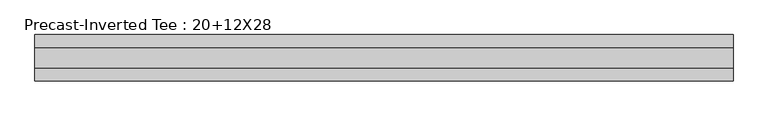
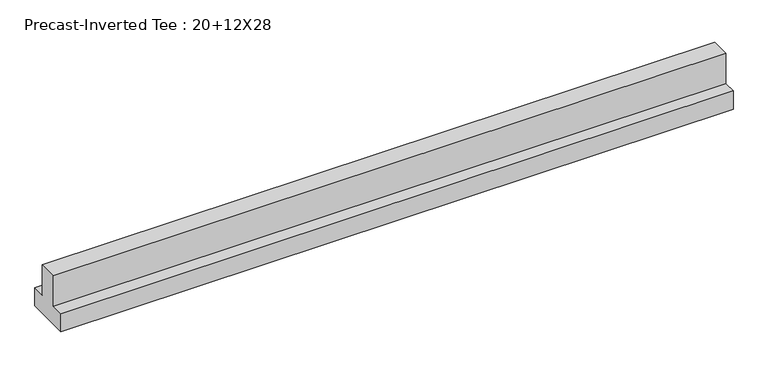
"""IFC4 building model written with IfcOpenShell, lengths in millimetres: beam geometry, Precast-Inverted Tee : 20+12X28."""

from ifc_helpers import new_model, si_unit, frame, origin, place, context, project, spatial, polyline, outline, extrude, source, transform, mapped, element, save


def precast_inverted_tee_20_12x28_9dfceafc(model_context):
    return source(origin(), model_context, "Body", "SweptSolid", [
        extrude(outline(polyline([(355.6, -406.4), (-355.6, -406.4), (-355.6, -101.6), (-152.4, -101.6), (-152.4, 406.4), (152.4, 406.4), (152.4, -101.6), (355.6, -101.6), (355.6, -406.4)])), frame((-5372.1, 0.0, 0.0), z_axis=(1.0, 0.0, 0.0), x_axis=(0.0, 1.0, 0.0)), (0.0, 0.0, 1.0), 10668.0),
    ])


if __name__ == "__main__":
    model = new_model("IFC4")
    model_context = context("Model", 3, world=origin())
    ifc_project = project(units=[si_unit("LENGTHUNIT", "METRE", prefix="MILLI")], contexts=[model_context])
    site = spatial("IfcSite", under=ifc_project)
    building = spatial("IfcBuilding", under=site)
    placement = place(None, origin())
    precast_inverted_tee_20_12x28_shape = precast_inverted_tee_20_12x28_9dfceafc(model_context)
    element("IfcBeam", 1, ObjectType="Precast-Inverted Tee : 20+12X28", at=placement, inside=building, context=model_context, shape_type="MappedRepresentation", body=[
        mapped(precast_inverted_tee_20_12x28_shape, transform((0.0, 0.0, 0.0), x_axis=(1.0, 0.0, 0.0), y_axis=(0.0, 1.0, 0.0), z_axis=(0.0, 0.0, 1.0))),
    ])
    save(model, "model.ifc")

# Revit data of these elements
# Type "Precast-Inverted Tee : 20+12X28"
#   Assembly Code = "B10"
#   Seat = 0' - 8"
#   Length [instance default] = 5' - 0"
#   b = 2' - 4"
#   h = 2' - 8"
#   h1 = 1' - 8"
#   Structural Material [instance default] = Concrete - Precast Concrete - Normal Weight Concrete - 5 ksi
# Element 1 (IfcBeam, "Precast-Inverted Tee : 20+12X28")
#   Length = 35' - 3"
#   Materials on its faces: "Concrete - Precast Concrete - Normal Weight Concrete - 5 ksi"
# Materials
#   "Concrete - Precast Concrete - Normal Weight Concrete - 5 ksi": class "Concrete", colour RGB 198 187 187, transparency 0, Cost = 0
